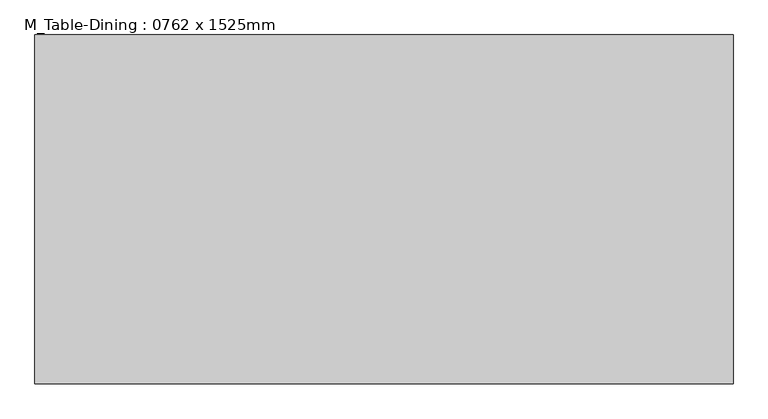
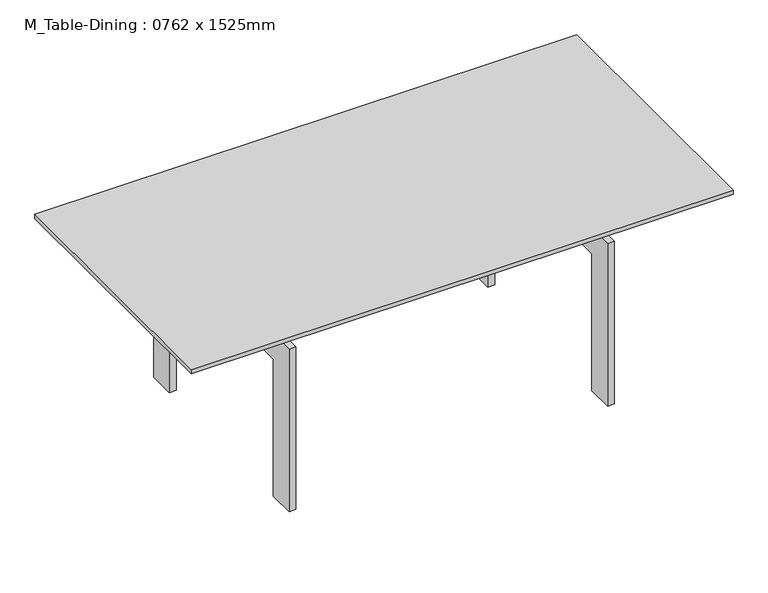
"""IFC4 building model written with IfcOpenShell, lengths in millimetres: furniture geometry, M_Table-Dining : 0762 x 1525mm."""

from ifc_helpers import new_model, si_unit, frame, origin, place, context, project, spatial, polyline, outline, extrude, source, transform, mapped, element, save


def m_table_dining_0762_x_1525mm_a1e3a7ba(model_context):
    return source(origin(), model_context, "Body", "SweptSolid", [
        extrude(outline(polyline([(679.1657667, 297.7823857), (679.1657667, 272.3823857), (-642.6342333, 272.3823857), (-642.6342333, 297.7823857), (679.1657667, 297.7823857)])), frame((0.0, 0.0, 483.8), z_axis=(0.0, 0.0, 1.0), x_axis=(1.0, 0.0, 0.0)), (0.0, 0.0, 1.0), 63.5),
        extrude(outline(polyline([(679.1657667, -82.5889222), (679.1657667, -107.9889222), (-642.6342333, -107.9889222), (-642.6342333, -82.5889222), (679.1657667, -82.5889222)])), frame((0.0, 0.0, 483.8), z_axis=(0.0, 0.0, 1.0), x_axis=(1.0, 0.0, 0.0)), (0.0, 0.0, 1.0), 63.5),
        extrude(outline(polyline([(425.4110778, 0.0), (349.2110778, 0.0), (349.2110778, 407.6), (-158.7889222, 407.6), (-158.7889222, 0.0), (-234.9889222, 0.0), (-234.9889222, 483.8), (425.4110778, 483.8), (425.4110778, 0.0)])), frame((456.9157667, 0.0, 0.0), z_axis=(1.0, 0.0, 0.0), x_axis=(0.0, 1.0, 0.0)), (0.0, 0.0, 1.0), 19.05),
        extrude(outline(polyline([(425.4110778, 483.8), (425.4110778, 0.0), (349.2110778, 0.0), (349.2110778, 407.6), (-158.7889222, 407.6), (-158.7889222, 0.0), (-234.9889222, 0.0), (-234.9889222, 483.8), (425.4110778, 483.8)])), frame((-439.4342333, 0.0, 0.0), z_axis=(1.0, 0.0, 0.0), x_axis=(0.0, 1.0, 0.0)), (0.0, 0.0, 1.0), 19.05),
        extrude(outline(polyline([(780.7657667, 476.2110778), (780.7657667, -285.7889222), (-744.2342333, -285.7889222), (-744.2342333, 476.2110778), (780.7657667, 476.2110778)])), frame((0.0, 0.0, 547.3), z_axis=(0.0, 0.0, 1.0), x_axis=(1.0, 0.0, 0.0)), (0.0, 0.0, 1.0), 12.7),
    ])


if __name__ == "__main__":
    model = new_model("IFC4")
    model_context = context("Model", 3, world=origin())
    ifc_project = project(units=[si_unit("LENGTHUNIT", "METRE", prefix="MILLI")], contexts=[model_context])
    site = spatial("IfcSite", under=ifc_project)
    building = spatial("IfcBuilding", under=site)
    placement = place(None, origin())
    m_table_dining_0762_x_1525mm_shape = m_table_dining_0762_x_1525mm_a1e3a7ba(model_context)
    element("IfcFurniture", 1, ObjectType="M_Table-Dining : 0762 x 1525mm", at=placement, inside=building, context=model_context, shape_type="MappedRepresentation", body=[
        mapped(m_table_dining_0762_x_1525mm_shape, transform((0.0, 0.0, 0.0), x_axis=(1.0, 0.0, 0.0), y_axis=(0.0, 1.0, 0.0), z_axis=(0.0, 0.0, 1.0))),
    ])
    save(model, "model.ifc")

# Revit data of these elements
# Type "M_Table-Dining : 0762 x 1525mm"
#   Height = 560 mm
#   Length = 1525 mm
#   Width = 762 mm
#   Base Material = Steel, Chrome Plated
#   Top Material = Glass - Clear, Grey
#   Default Elevation = 0
# Element 1 (IfcFurniture, "M_Table-Dining : 0762 x 1525mm")
#   Materials on its faces: "Steel, Chrome Plated", "Glass - Clear, Grey"
# Materials
#   "Steel, Chrome Plated": class "Metal", colour RGB 17 17 17, transparency 0, Description = "Chromiuim plated steel", Cost = 0
#   "Glass - Clear, Grey": class "Glass", colour RGB 252 255 255, transparency 0.64
